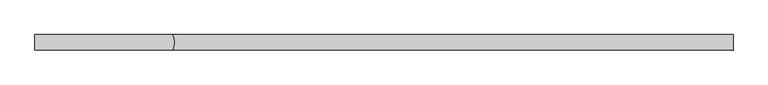
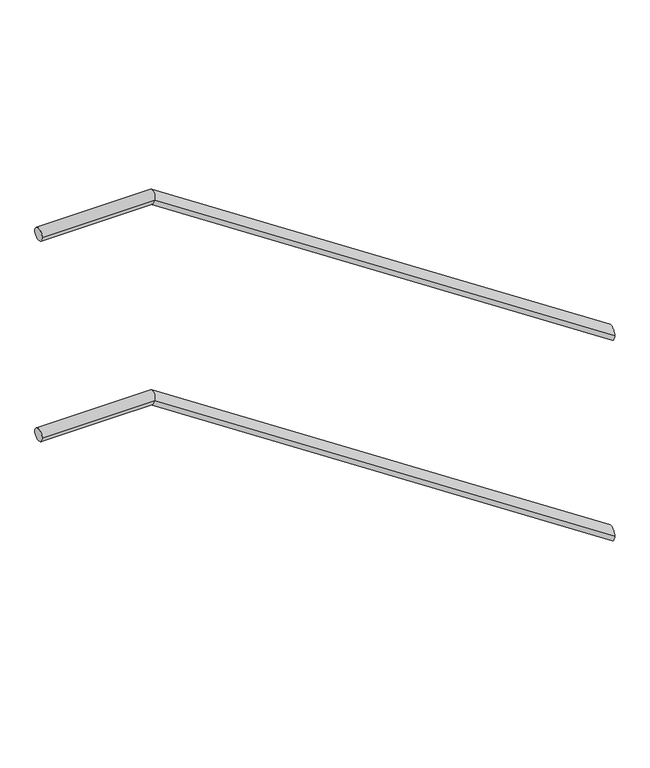
"""IFC4 building model written with IfcOpenShell, lengths in millimetres: railing geometry."""

from ifc_helpers import new_model, si_unit, frame, origin, place, context, project, spatial, circle_curve, ellipse_curve, source, transform, mapped, element, save
from ifc_brep_helpers import plane_surface, cylinder_surface, advanced_brep


def railing_36ed9c91(model_context):
    return source(origin(), model_context, "Body", "AdvancedBrep", [
        advanced_brep(
        [(48078.2332408, 8219.6306666, 910.5875748), (48078.2332408, 8249.6306666, 910.5875748), (46993.7216539, 8219.6306666, 1627.8571429), (46993.7216539, 8249.6306666, 1627.8571429), (46728.2332408, 8219.6306666, 1627.8571429), (46728.2332408, 8249.6306666, 1627.8571429)],
        [
            (0, 1, ellipse_curve(frame((48078.2332408, 8234.6306666, 910.5875748), z_axis=(1.0, 0.0, 0.0), x_axis=(0.0, 0.0, -1.0)), 17.9838538, 15.0)),
            (1, 0, ellipse_curve(frame((48078.2332408, 8234.6306666, 910.5875748), z_axis=(1.0, 0.0, 0.0), x_axis=(0.0, 0.0, -1.0)), 17.9838538, 15.0)),
            (0, 2),
            (2, 3, ellipse_curve(frame((46993.7216539, 8234.6306666, 1627.8571429), z_axis=(0.9576224501515418, 0.0, -0.28802646226650325), x_axis=(-0.288026462266502, 0.0, -0.9576224501515423)), 15.6637932, 15.0)),
            (3, 1),
            (3, 2, ellipse_curve(frame((46993.7216539, 8234.6306666, 1627.8571429), z_axis=(0.9576224501515418, 0.0, -0.28802646226650325), x_axis=(-0.288026462266502, 0.0, -0.9576224501515423)), 15.6637932, 15.0)),
            (4, 5, circle_curve(frame((46728.2332408, 8234.6306666, 1627.8571429), z_axis=(-1.0, 0.0, 0.0), x_axis=(0.0, 1.0, 0.0)), 15.0)),
            (5, 4, circle_curve(frame((46728.2332408, 8234.6306666, 1627.8571429), z_axis=(-1.0, 0.0, 0.0), x_axis=(0.0, 1.0, 0.0)), 15.0)),
            (2, 4),
            (5, 3),
        ],
        [
            plane_surface(frame((48078.2332408, 8234.6306666, 928.5714286), z_axis=(1.0, 0.0, 0.0), x_axis=(0.0, -1.0, 0.0))),
            cylinder_surface(frame((48069.9586226, 8234.6306666, 916.0602059), z_axis=(0.8340815140684851, 0.0, -0.5516412130082591), x_axis=(0.0, 1.0, 0.0)), 15.0),
            plane_surface(frame((46728.2332408, 8234.6306666, 1642.8571429), z_axis=(-1.0, 0.0, 0.0), x_axis=(0.0, -1.0, 0.0))),
            cylinder_surface(frame((46998.2332408, 8234.6306666, 1627.8571429), z_axis=(1.0, 0.0, 0.0), x_axis=(0.0, 1.0, 0.0)), 15.0),
        ],
        [
            (0, [[1, 2]]),
            (1, [[-1, 3, 4, 5]]),
            (1, [[-2, -5, 6, -3]]),
            (2, [[7, 8]]),
            (3, [[-4, 9, -8, 10]]),
            (3, [[-6, -10, -7, -9]]),
        ],
    ),
        advanced_brep(
        [(48078.2332408, 8219.6306666, 1410.5875748), (48078.2332408, 8249.6306666, 1410.5875748), (46993.7216539, 8219.6306666, 2127.8571429), (46993.7216539, 8249.6306666, 2127.8571429), (46728.2332408, 8219.6306666, 2127.8571429), (46728.2332408, 8249.6306666, 2127.8571429)],
        [
            (0, 1, ellipse_curve(frame((48078.2332408, 8234.6306666, 1410.5875748), z_axis=(1.0, 0.0, 0.0), x_axis=(0.0, 0.0, -1.0)), 17.9838538, 15.0)),
            (1, 0, ellipse_curve(frame((48078.2332408, 8234.6306666, 1410.5875748), z_axis=(1.0, 0.0, 0.0), x_axis=(0.0, 0.0, -1.0)), 17.9838538, 15.0)),
            (0, 2),
            (2, 3, ellipse_curve(frame((46993.7216539, 8234.6306666, 2127.8571429), z_axis=(0.9576224501515418, 0.0, -0.28802646226650325), x_axis=(-0.288026462266502, 0.0, -0.9576224501515423)), 15.6637932, 15.0)),
            (3, 1),
            (3, 2, ellipse_curve(frame((46993.7216539, 8234.6306666, 2127.8571429), z_axis=(0.9576224501515418, 0.0, -0.28802646226650325), x_axis=(-0.288026462266502, 0.0, -0.9576224501515423)), 15.6637932, 15.0)),
            (4, 5, circle_curve(frame((46728.2332408, 8234.6306666, 2127.8571429), z_axis=(-1.0, 0.0, 0.0), x_axis=(0.0, 1.0, 0.0)), 15.0)),
            (5, 4, circle_curve(frame((46728.2332408, 8234.6306666, 2127.8571429), z_axis=(-1.0, 0.0, 0.0), x_axis=(0.0, 1.0, 0.0)), 15.0)),
            (2, 4),
            (5, 3),
        ],
        [
            plane_surface(frame((48078.2332408, 8234.6306666, 1428.5714286), z_axis=(1.0, 0.0, 0.0), x_axis=(0.0, -1.0, 0.0))),
            cylinder_surface(frame((48069.9586226, 8234.6306666, 1416.0602059), z_axis=(0.8340815140684851, 0.0, -0.5516412130082591), x_axis=(0.0, 1.0, 0.0)), 15.0),
            plane_surface(frame((46728.2332408, 8234.6306666, 2142.8571429), z_axis=(-1.0, 0.0, 0.0), x_axis=(0.0, -1.0, 0.0))),
            cylinder_surface(frame((46998.2332408, 8234.6306666, 2127.8571429), z_axis=(1.0, 0.0, 0.0), x_axis=(0.0, 1.0, 0.0)), 15.0),
        ],
        [
            (0, [[1, 2]]),
            (1, [[-1, 3, 4, 5]]),
            (1, [[-2, -5, 6, -3]]),
            (2, [[7, 8]]),
            (3, [[-4, 9, -8, 10]]),
            (3, [[-6, -10, -7, -9]]),
        ],
    ),
    ])


if __name__ == "__main__":
    model = new_model("IFC4")
    model_context = context("Model", 3, world=origin())
    ifc_project = project(units=[si_unit("LENGTHUNIT", "METRE", prefix="MILLI")], contexts=[model_context])
    site = spatial("IfcSite", under=ifc_project)
    building = spatial("IfcBuilding", under=site)
    placement = place(None, origin())
    railing_shape = railing_36ed9c91(model_context)
    element("IfcRailing", 1, at=placement, inside=building, context=model_context, shape_type="MappedRepresentation", body=[
        mapped(railing_shape, transform((0.0, 0.0, 0.0), x_axis=(1.0, 0.0, 0.0), y_axis=(0.0, 1.0, 0.0), z_axis=(0.0, 0.0, 1.0))),
    ])
    save(model, "model.ifc")
